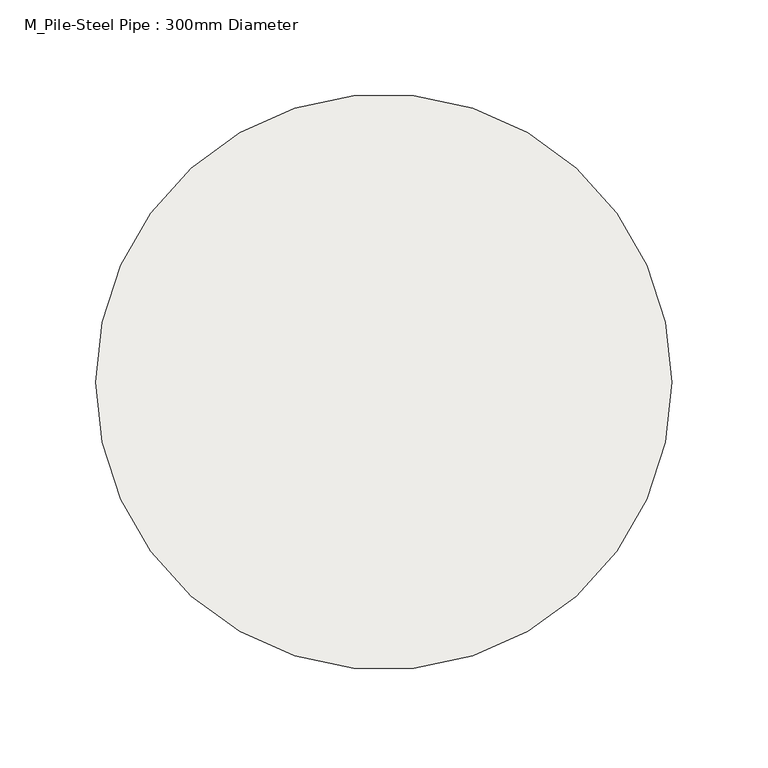
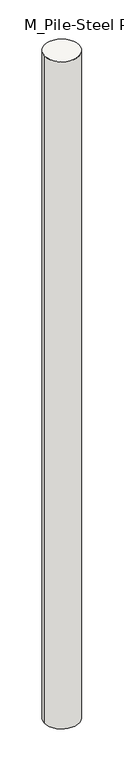
"""IFC4 building model written with IfcOpenShell, lengths in millimetres: slab geometry, M_Pile-Steel Pipe : 300mm Diameter."""

import ifcopenshell
import ifcopenshell.guid

model = None  # the IFC model being written
_history = None  # IfcOwnerHistory: only IFC2X3 demands one
_inside = {}  # id of a spatial element -> (the spatial element, [elements in it])
_under = {}  # id of a project, library or spatial element -> (it, [spatial elements below it])
_declared = {}  # id of a project -> (the project, [libraries it declares])
_typed = {}  # id of a type object -> (the type object, [elements of that type])
_made_of = {}  # id of a material, layer set ... -> (it, [elements and type objects made of it])


def new_model(schema):
    """Start an empty IFC model of exactly this schema.

    Asked for "IFC4X3", IfcOpenShell would pick the latest addendum, in which some entities
    have other attributes; the version numbers below select the first issue.
    IFC2X3 requires an IfcOwnerHistory on every rooted entity: one is made here for all.
    """
    global model, _history
    if schema == "IFC4X3":
        model = ifcopenshell.file(schema_version=(4, 3, 0, 0))
    else:
        model = ifcopenshell.file(schema=schema)
    _inside.clear()
    _under.clear()
    _declared.clear()
    _typed.clear()
    _made_of.clear()
    _history = None
    if model.schema == "IFC2X3":
        org = make("IfcOrganization", Name="unknown")
        user = make(
            "IfcPersonAndOrganization",
            ThePerson=make("IfcPerson", FamilyName="unknown"),
            TheOrganization=org,
        )
        app = make(
            "IfcApplication",
            ApplicationDeveloper=org,
            Version="unknown",
            ApplicationFullName="unknown",
            ApplicationIdentifier="unknown",
        )
        _history = make(
            "IfcOwnerHistory",
            OwningUser=user,
            OwningApplication=app,
            ChangeAction="ADDED",
            CreationDate=0,
        )
    return model


def make(cls, **values):
    """One entity of the class cls with the attributes given. An attribute that is None is left unset."""
    return model.create_entity(
        cls, **{name: value for name, value in values.items() if value is not None}
    )


def rooted(cls, **values):
    """An entity with a GlobalId (a new one), such as an element, a storey or a relation."""
    return make(cls, GlobalId=ifcopenshell.guid.new(), OwnerHistory=_history, **values)


def si_unit(unit_type, name, prefix=None):
    """IfcSIUnit, for example si_unit("LENGTHUNIT", "METRE", prefix="MILLI")."""
    return make("IfcSIUnit", UnitType=unit_type, Prefix=prefix, Name=name)


def assignment(units):
    """IfcUnitAssignment: the units of a project."""
    return None if units is None else make("IfcUnitAssignment", Units=units)


def point(xyz):
    """IfcCartesianPoint."""
    return None if xyz is None else make("IfcCartesianPoint", Coordinates=xyz)


def direction(xyz):
    """IfcDirection."""
    return None if xyz is None else make("IfcDirection", DirectionRatios=xyz)


def frame(location, z_axis=None, x_axis=None):
    """IfcAxis2Placement3D, a coordinate frame: its origin and axes. An axis left out is left unset."""
    return make(
        "IfcAxis2Placement3D",
        Location=point(location),
        Axis=direction(z_axis),
        RefDirection=direction(x_axis),
    )


def frame_2d(location, x_axis=None):
    """IfcAxis2Placement2D, a coordinate frame in the plane: its origin and x axis."""
    return make(
        "IfcAxis2Placement2D", Location=point(location), RefDirection=direction(x_axis)
    )


def origin():
    """The frame at (0, 0, 0) with its axes left unset."""
    return frame((0.0, 0.0, 0.0))


def origin_2d():
    """The frame at (0, 0) in the plane with its x axis left unset."""
    return frame_2d((0.0, 0.0))


def place(relative_to, where):
    """IfcLocalPlacement: puts the frame where relative to a parent placement (None: the world)."""
    return make(
        "IfcLocalPlacement", PlacementRelTo=relative_to, RelativePlacement=where
    )


def context(
    kind, dimensions, precision=None, world=None, true_north=None, identifier=None
):
    """IfcGeometricRepresentationContext, for example the 3D "Model" context."""
    return make(
        "IfcGeometricRepresentationContext",
        ContextIdentifier=identifier,
        ContextType=kind,
        CoordinateSpaceDimension=dimensions,
        Precision=precision,
        WorldCoordinateSystem=world,
        TrueNorth=true_north,
    )


def project(units=None, contexts=None):
    """IfcProject with its units and contexts."""
    return rooted(
        "IfcProject",
        Name="project",
        RepresentationContexts=contexts,
        UnitsInContext=assignment(units),
    )


def spatial(cls, under=None, at=None, **own):
    """A site, building, storey or space (cls), placed at a placement, below another one or the project."""
    s = rooted(cls, ObjectPlacement=at, **own)
    if under is not None:
        _under.setdefault(under.id(), (under, []))[1].append(s)
    return s


def circle_curve(where, radius):
    """IfcCircle in the frame where."""
    return make("IfcCircle", Position=where, Radius=radius)


def trimmed(basis, trim1, trim2, sense, master):
    """IfcTrimmedCurve: the piece of a basis curve between two trims."""
    return make(
        "IfcTrimmedCurve",
        BasisCurve=basis,
        Trim1=trim1,
        Trim2=trim2,
        SenseAgreement=sense,
        MasterRepresentation=master,
    )


def segment(curve, same_sense, transition):
    """IfcCompositeCurveSegment."""
    return make(
        "IfcCompositeCurveSegment",
        Transition=transition,
        SameSense=same_sense,
        ParentCurve=curve,
    )


def composite_curve(segments, self_intersect=None):
    """IfcCompositeCurve: segments joined end to end."""
    return make("IfcCompositeCurve", Segments=segments, SelfIntersect=self_intersect)


def outline(outer, holes=None, kind="AREA"):
    """IfcArbitraryClosedProfileDef: a profile drawn as a closed curve; with holes, ...WithVoids."""
    if holes is None:
        return make("IfcArbitraryClosedProfileDef", ProfileType=kind, OuterCurve=outer)
    return make(
        "IfcArbitraryProfileDefWithVoids",
        ProfileType=kind,
        OuterCurve=outer,
        InnerCurves=holes,
    )


def extrude(swept, where, along, depth):
    """IfcExtrudedAreaSolid: the profile swept, set in the frame where, extruded along a direction by depth."""
    return make(
        "IfcExtrudedAreaSolid",
        SweptArea=swept,
        Position=where,
        ExtrudedDirection=direction(along),
        Depth=depth,
    )


def shape(context_of_items, identifier, shape_type, items):
    """IfcShapeRepresentation: the items that make up one representation, for example the "Body"."""
    return make(
        "IfcShapeRepresentation",
        ContextOfItems=context_of_items,
        RepresentationIdentifier=identifier,
        RepresentationType=shape_type,
        Items=items,
    )


def source(mapping_origin, context_of_items, identifier, shape_type, items):
    """IfcRepresentationMap: a shape defined once, which mapped items show again and again."""
    return make(
        "IfcRepresentationMap",
        MappingOrigin=mapping_origin,
        MappedRepresentation=shape(context_of_items, identifier, shape_type, items),
    )


def transform(
    local_origin,
    x_axis=None,
    y_axis=None,
    z_axis=None,
    scale=None,
    scale2=None,
    scale3=None,
    uniform=True,
):
    """IfcCartesianTransformationOperator3D, or its non-uniform kind. x_axis, y_axis, z_axis: its Axis1, 2, 3."""
    if uniform:
        return make(
            "IfcCartesianTransformationOperator3D",
            Axis1=direction(x_axis),
            Axis2=direction(y_axis),
            LocalOrigin=point(local_origin),
            Scale=scale,
            Axis3=direction(z_axis),
        )
    return make(
        "IfcCartesianTransformationOperator3DnonUniform",
        Axis1=direction(x_axis),
        Axis2=direction(y_axis),
        LocalOrigin=point(local_origin),
        Scale=scale,
        Axis3=direction(z_axis),
        Scale2=scale2,
        Scale3=scale3,
    )


def mapped(mapping_source, mapping_target):
    """IfcMappedItem: shows the shape of a source again, moved by a transform."""
    return make(
        "IfcMappedItem", MappingSource=mapping_source, MappingTarget=mapping_target
    )


def made_of(thing, what):
    """Note that an element or type object is made of a material, layer set ...; save() writes the relation."""
    if what is not None:
        _made_of.setdefault(what.id(), (what, []))[1].append(thing)
    return thing


def element(
    cls,
    number,
    at=None,
    inside=None,
    cuts=None,
    type_object=None,
    material=None,
    context=None,
    identifier="Body",
    shape_type=None,
    held_by="IfcProductDefinitionShape",
    body=None,
    shapes=None,
    **own,
):
    """One element of the class cls, such as IfcWall. Its Tag is "e" and its number.

    at: its placement. inside: the storey or other place that contains it. cuts: it is an
    opening in that element (IfcRelVoidsElement). A single representation is given by context,
    identifier, shape_type and body (its items); several are given by shapes. held_by: the class
    of the entity that holds the representations. save() writes the other relations.
    """
    e = rooted(cls, Tag="e%d" % number, ObjectPlacement=at, **own)
    if body is not None:
        shapes = [shape(context, identifier, shape_type, body)]
    if shapes is not None:
        e.Representation = make(held_by, Representations=shapes)
    if inside is not None:
        _inside.setdefault(inside.id(), (inside, []))[1].append(e)
    if cuts is not None:
        rooted(
            "IfcRelVoidsElement", RelatingBuildingElement=cuts, RelatedOpeningElement=e
        )
    if type_object is not None:
        _typed.setdefault(type_object.id(), (type_object, []))[1].append(e)
    return made_of(e, material)


def aggregate(whole, parts):
    """IfcRelAggregates: a whole, such as a stair, and the parts it consists of."""
    return rooted("IfcRelAggregates", RelatingObject=whole, RelatedObjects=parts)


def save(model, path):
    """Write the relations noted so far, then the file.

    IfcRelAggregates (storeys below a building ...), IfcRelContainedInSpatialStructure (elements
    in a storey), IfcRelDefinesByType, IfcRelAssociatesMaterial and IfcRelDeclares: one each for
    every whole, place, type object, material and project.
    """
    for whole, parts in _under.values():
        aggregate(whole, parts)
    for where, things in _inside.values():
        rooted(
            "IfcRelContainedInSpatialStructure",
            RelatedElements=things,
            RelatingStructure=where,
        )
    for kind, things in _typed.values():
        rooted("IfcRelDefinesByType", RelatedObjects=things, RelatingType=kind)
    for what, things in _made_of.values():
        rooted("IfcRelAssociatesMaterial", RelatedObjects=things, RelatingMaterial=what)
    for by, libraries in _declared.values():
        rooted("IfcRelDeclares", RelatingContext=by, RelatedDefinitions=libraries)
    model.write(path)


def m_pile_steel_pipe_300mm_diameter_9db3f09c(model_context):
    return source(origin(), model_context, "Body", "SweptSolid", [
        extrude(outline(composite_curve([segment(trimmed(circle_curve(origin_2d(), 150.0), [point((-150.0, 0.0))], [point((150.0, 0.0))], False, "CARTESIAN"), True, "CONTINUOUS"), segment(trimmed(circle_curve(origin_2d(), 150.0), [point((150.0, 0.0))], [point((-150.0, 0.0))], False, "CARTESIAN"), True, "CONTINUOUS")], self_intersect=False)), frame((0.0, 0.0, -6000.0), z_axis=(0.0, 0.0, 1.0), x_axis=(1.0, 0.0, 0.0)), (0.0, 0.0, 1.0), 6150.0),
    ])


if __name__ == "__main__":
    model = new_model("IFC4")
    model_context = context("Model", 3, world=origin())
    ifc_project = project(units=[si_unit("LENGTHUNIT", "METRE", prefix="MILLI")], contexts=[model_context])
    site = spatial("IfcSite", under=ifc_project)
    building = spatial("IfcBuilding", under=site)
    placement = place(None, origin())
    m_pile_steel_pipe_300mm_diameter_shape = m_pile_steel_pipe_300mm_diameter_9db3f09c(model_context)
    element("IfcSlab", 1, ObjectType="M_Pile-Steel Pipe : 300mm Diameter", at=placement, inside=building, context=model_context, shape_type="MappedRepresentation", body=[
        mapped(m_pile_steel_pipe_300mm_diameter_shape, transform((0.0, 0.0, 0.0), x_axis=(1.0, 0.0, 0.0), y_axis=(0.0, 1.0, 0.0), z_axis=(0.0, 0.0, 1.0))),
    ])
    save(model, "model.ifc")

# Revit data of these elements
# Type "M_Pile-Steel Pipe : 300mm Diameter"
#   Assembly Code = "A1020130"
#   Radius = 150 mm
#   Minimum Embedment = 150 mm
#   Diameter = 300 mm
#   Depth = 6000 mm
#   Structural Material [instance default] = Steel, 45-345
# Element 1 (IfcSlab, "M_Pile-Steel Pipe : 300mm Diameter")
#   Materials on its faces: "Steel, 45-345"
# Materials
#   "Steel, 45-345": class "Metal", colour RGB 247 247 247, transparency 0, Description = "Steel 345 MPa", Cost = 0
